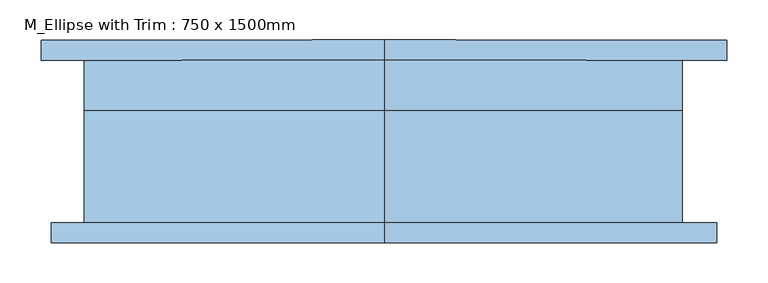
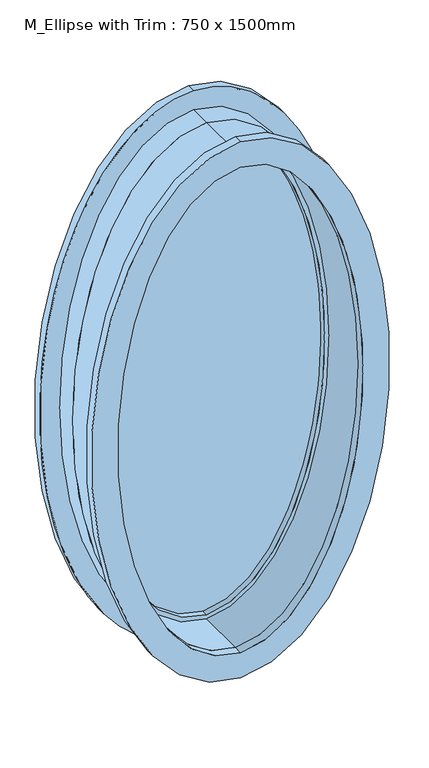
"""IFC4 building model written with IfcOpenShell, lengths in millimetres: window geometry, M_Ellipse with Trim : 750 x 1500mm."""

import ifcopenshell
import ifcopenshell.guid

model = None  # the IFC model being written
_history = None  # IfcOwnerHistory: only IFC2X3 demands one
_inside = {}  # id of a spatial element -> (the spatial element, [elements in it])
_under = {}  # id of a project, library or spatial element -> (it, [spatial elements below it])
_declared = {}  # id of a project -> (the project, [libraries it declares])
_typed = {}  # id of a type object -> (the type object, [elements of that type])
_made_of = {}  # id of a material, layer set ... -> (it, [elements and type objects made of it])


def new_model(schema):
    """Start an empty IFC model of exactly this schema.

    Asked for "IFC4X3", IfcOpenShell would pick the latest addendum, in which some entities
    have other attributes; the version numbers below select the first issue.
    IFC2X3 requires an IfcOwnerHistory on every rooted entity: one is made here for all.
    """
    global model, _history
    if schema == "IFC4X3":
        model = ifcopenshell.file(schema_version=(4, 3, 0, 0))
    else:
        model = ifcopenshell.file(schema=schema)
    _inside.clear()
    _under.clear()
    _declared.clear()
    _typed.clear()
    _made_of.clear()
    _history = None
    if model.schema == "IFC2X3":
        org = make("IfcOrganization", Name="unknown")
        user = make(
            "IfcPersonAndOrganization",
            ThePerson=make("IfcPerson", FamilyName="unknown"),
            TheOrganization=org,
        )
        app = make(
            "IfcApplication",
            ApplicationDeveloper=org,
            Version="unknown",
            ApplicationFullName="unknown",
            ApplicationIdentifier="unknown",
        )
        _history = make(
            "IfcOwnerHistory",
            OwningUser=user,
            OwningApplication=app,
            ChangeAction="ADDED",
            CreationDate=0,
        )
    return model


def make(cls, **values):
    """One entity of the class cls with the attributes given. An attribute that is None is left unset."""
    return model.create_entity(
        cls, **{name: value for name, value in values.items() if value is not None}
    )


def rooted(cls, **values):
    """An entity with a GlobalId (a new one), such as an element, a storey or a relation."""
    return make(cls, GlobalId=ifcopenshell.guid.new(), OwnerHistory=_history, **values)


def si_unit(unit_type, name, prefix=None):
    """IfcSIUnit, for example si_unit("LENGTHUNIT", "METRE", prefix="MILLI")."""
    return make("IfcSIUnit", UnitType=unit_type, Prefix=prefix, Name=name)


def assignment(units):
    """IfcUnitAssignment: the units of a project."""
    return None if units is None else make("IfcUnitAssignment", Units=units)


def point(xyz):
    """IfcCartesianPoint."""
    return None if xyz is None else make("IfcCartesianPoint", Coordinates=xyz)


def direction(xyz):
    """IfcDirection."""
    return None if xyz is None else make("IfcDirection", DirectionRatios=xyz)


def frame(location, z_axis=None, x_axis=None):
    """IfcAxis2Placement3D, a coordinate frame: its origin and axes. An axis left out is left unset."""
    return make(
        "IfcAxis2Placement3D",
        Location=point(location),
        Axis=direction(z_axis),
        RefDirection=direction(x_axis),
    )


def origin():
    """The frame at (0, 0, 0) with its axes left unset."""
    return frame((0.0, 0.0, 0.0))


def place(relative_to, where):
    """IfcLocalPlacement: puts the frame where relative to a parent placement (None: the world)."""
    return make(
        "IfcLocalPlacement", PlacementRelTo=relative_to, RelativePlacement=where
    )


def context(
    kind, dimensions, precision=None, world=None, true_north=None, identifier=None
):
    """IfcGeometricRepresentationContext, for example the 3D "Model" context."""
    return make(
        "IfcGeometricRepresentationContext",
        ContextIdentifier=identifier,
        ContextType=kind,
        CoordinateSpaceDimension=dimensions,
        Precision=precision,
        WorldCoordinateSystem=world,
        TrueNorth=true_north,
    )


def project(units=None, contexts=None):
    """IfcProject with its units and contexts."""
    return rooted(
        "IfcProject",
        Name="project",
        RepresentationContexts=contexts,
        UnitsInContext=assignment(units),
    )


def spatial(cls, under=None, at=None, **own):
    """A site, building, storey or space (cls), placed at a placement, below another one or the project."""
    s = rooted(cls, ObjectPlacement=at, **own)
    if under is not None:
        _under.setdefault(under.id(), (under, []))[1].append(s)
    return s


def ellipse_curve(where, semi_axis1, semi_axis2):
    """IfcEllipse in the frame where."""
    return make(
        "IfcEllipse", Position=where, SemiAxis1=semi_axis1, SemiAxis2=semi_axis2
    )


def trimmed(basis, trim1, trim2, sense, master):
    """IfcTrimmedCurve: the piece of a basis curve between two trims."""
    return make(
        "IfcTrimmedCurve",
        BasisCurve=basis,
        Trim1=trim1,
        Trim2=trim2,
        SenseAgreement=sense,
        MasterRepresentation=master,
    )


def shape(context_of_items, identifier, shape_type, items):
    """IfcShapeRepresentation: the items that make up one representation, for example the "Body"."""
    return make(
        "IfcShapeRepresentation",
        ContextOfItems=context_of_items,
        RepresentationIdentifier=identifier,
        RepresentationType=shape_type,
        Items=items,
    )


def source(mapping_origin, context_of_items, identifier, shape_type, items):
    """IfcRepresentationMap: a shape defined once, which mapped items show again and again."""
    return make(
        "IfcRepresentationMap",
        MappingOrigin=mapping_origin,
        MappedRepresentation=shape(context_of_items, identifier, shape_type, items),
    )


def transform(
    local_origin,
    x_axis=None,
    y_axis=None,
    z_axis=None,
    scale=None,
    scale2=None,
    scale3=None,
    uniform=True,
):
    """IfcCartesianTransformationOperator3D, or its non-uniform kind. x_axis, y_axis, z_axis: its Axis1, 2, 3."""
    if uniform:
        return make(
            "IfcCartesianTransformationOperator3D",
            Axis1=direction(x_axis),
            Axis2=direction(y_axis),
            LocalOrigin=point(local_origin),
            Scale=scale,
            Axis3=direction(z_axis),
        )
    return make(
        "IfcCartesianTransformationOperator3DnonUniform",
        Axis1=direction(x_axis),
        Axis2=direction(y_axis),
        LocalOrigin=point(local_origin),
        Scale=scale,
        Axis3=direction(z_axis),
        Scale2=scale2,
        Scale3=scale3,
    )


def mapped(mapping_source, mapping_target):
    """IfcMappedItem: shows the shape of a source again, moved by a transform."""
    return make(
        "IfcMappedItem", MappingSource=mapping_source, MappingTarget=mapping_target
    )


def made_of(thing, what):
    """Note that an element or type object is made of a material, layer set ...; save() writes the relation."""
    if what is not None:
        _made_of.setdefault(what.id(), (what, []))[1].append(thing)
    return thing


def element(
    cls,
    number,
    at=None,
    inside=None,
    cuts=None,
    type_object=None,
    material=None,
    context=None,
    identifier="Body",
    shape_type=None,
    held_by="IfcProductDefinitionShape",
    body=None,
    shapes=None,
    **own,
):
    """One element of the class cls, such as IfcWall. Its Tag is "e" and its number.

    at: its placement. inside: the storey or other place that contains it. cuts: it is an
    opening in that element (IfcRelVoidsElement). A single representation is given by context,
    identifier, shape_type and body (its items); several are given by shapes. held_by: the class
    of the entity that holds the representations. save() writes the other relations.
    """
    e = rooted(cls, Tag="e%d" % number, ObjectPlacement=at, **own)
    if body is not None:
        shapes = [shape(context, identifier, shape_type, body)]
    if shapes is not None:
        e.Representation = make(held_by, Representations=shapes)
    if inside is not None:
        _inside.setdefault(inside.id(), (inside, []))[1].append(e)
    if cuts is not None:
        rooted(
            "IfcRelVoidsElement", RelatingBuildingElement=cuts, RelatedOpeningElement=e
        )
    if type_object is not None:
        _typed.setdefault(type_object.id(), (type_object, []))[1].append(e)
    return made_of(e, material)


def aggregate(whole, parts):
    """IfcRelAggregates: a whole, such as a stair, and the parts it consists of."""
    return rooted("IfcRelAggregates", RelatingObject=whole, RelatedObjects=parts)


def save(model, path):
    """Write the relations noted so far, then the file.

    IfcRelAggregates (storeys below a building ...), IfcRelContainedInSpatialStructure (elements
    in a storey), IfcRelDefinesByType, IfcRelAssociatesMaterial and IfcRelDeclares: one each for
    every whole, place, type object, material and project.
    """
    for whole, parts in _under.values():
        aggregate(whole, parts)
    for where, things in _inside.values():
        rooted(
            "IfcRelContainedInSpatialStructure",
            RelatedElements=things,
            RelatingStructure=where,
        )
    for kind, things in _typed.values():
        rooted("IfcRelDefinesByType", RelatedObjects=things, RelatingType=kind)
    for what, things in _made_of.values():
        rooted("IfcRelAssociatesMaterial", RelatedObjects=things, RelatingMaterial=what)
    for by, libraries in _declared.values():
        rooted("IfcRelDeclares", RelatingContext=by, RelatedDefinitions=libraries)
    model.write(path)


def plane_surface(at):
    """IfcPlane: the flat surface through the origin of the frame at, square to its z axis."""
    return make("IfcPlane", Position=at)


def extruded_surface(curve, direction_of_extrusion, depth):
    """IfcSurfaceOfLinearExtrusion: the curve pushed along a direction by depth."""
    return make(
        "IfcSurfaceOfLinearExtrusion",
        SweptCurve=make("IfcArbitraryOpenProfileDef", ProfileType="CURVE", Curve=curve),
        ExtrudedDirection=direction(direction_of_extrusion),
        Depth=depth,
    )


def advanced_brep(points, edges, surfaces, faces):
    """IfcAdvancedBrep: a solid bounded by faces that lie on surfaces and meet in shared edges.

    An edge is (start, end): straight between two places in points (the first is 0);
    or (start, end, curve); or (start, end, curve, False) where it runs against its curve.
    A face is (place in surfaces, loops), or (place, loops, False) where it looks against
    its surface's normal. A loop lists edges by number (the first is 1), with a minus sign
    where the edge is run from its end to its start. The first loop is the outer one.
    """
    corners = [point(p) for p in points]
    vertices = [make("IfcVertexPoint", VertexGeometry=c) for c in corners]
    made = []
    for start, end, *more in edges:
        made.append(
            make(
                "IfcEdgeCurve",
                EdgeStart=vertices[start],
                EdgeEnd=vertices[end],
                EdgeGeometry=more[0] if more else make("IfcPolyline", Points=[corners[start], corners[end]]),
                SameSense=more[1] if len(more) > 1 else True,
            )
        )
    hull = []
    for where, loops, *sense in faces:
        bounds = []
        for j, loop in enumerate(loops):
            ring = [make("IfcOrientedEdge", EdgeElement=made[abs(k) - 1], Orientation=k > 0) for k in loop]
            bounds.append(
                make(
                    "IfcFaceOuterBound" if j == 0 else "IfcFaceBound",
                    Bound=make("IfcEdgeLoop", EdgeList=ring),
                    Orientation=True,
                )
            )
        hull.append(make("IfcAdvancedFace", Bounds=bounds, FaceSurface=surfaces[where], SameSense=sense[0] if sense else True))
    return make("IfcAdvancedBrep", Outer=make("IfcClosedShell", CfsFaces=hull))


def m_ellipse_with_trim_750_x_1500mm_90dfdbfc(model_context):
    return source(origin(), model_context, "Body", "AdvancedBrep", [
        advanced_brep(
        [(0.0, -101.6, 2415.0), (0.0, -101.6, 915.0), (0.0, -101.6, 2383.25), (0.0, -101.6, 946.75), (0.0, 38.1, 2415.0), (0.0, 38.1, 915.0), (0.0, 38.1, 2383.25), (0.0, 38.1, 946.75)],
        [
            (0, 1, ellipse_curve(frame((0.0, -101.6, 1665.0), z_axis=(0.0, -1.0, 0.0), x_axis=(0.0, 0.0, -1.0)), 750.0, 375.0)),
            (1, 0, ellipse_curve(frame((0.0, -101.6, 1665.0), z_axis=(0.0, -1.0, 0.0), x_axis=(0.0, 0.0, -1.0)), 750.0, 375.0)),
            (2, 3, ellipse_curve(frame((0.0, -101.6, 1665.0), z_axis=(0.0, 1.0, 0.0), x_axis=(0.0, 0.0, -1.0)), 718.25, 343.25)),
            (3, 2, ellipse_curve(frame((0.0, -101.6, 1665.0), z_axis=(0.0, 1.0, 0.0), x_axis=(0.0, 0.0, -1.0)), 718.25, 343.25)),
            (0, 4),
            (4, 5, ellipse_curve(frame((0.0, 38.1, 1665.0), z_axis=(0.0, -1.0, 0.0), x_axis=(0.0, 0.0, -1.0)), 750.0, 375.0)),
            (5, 1),
            (5, 4, ellipse_curve(frame((0.0, 38.1, 1665.0), z_axis=(0.0, -1.0, 0.0), x_axis=(0.0, 0.0, -1.0)), 750.0, 375.0)),
            (2, 6),
            (6, 7, ellipse_curve(frame((0.0, 38.1, 1665.0), z_axis=(0.0, 1.0, 0.0), x_axis=(0.0, 0.0, -1.0)), 718.25, 343.25)),
            (7, 3),
            (7, 6, ellipse_curve(frame((0.0, 38.1, 1665.0), z_axis=(0.0, 1.0, 0.0), x_axis=(0.0, 0.0, -1.0)), 718.25, 343.25)),
        ],
        [
            plane_surface(frame((0.0, -101.6, 915.0), z_axis=(0.0, -1.0, 0.0), x_axis=(1.0, 0.0, 0.0))),
            extruded_surface(trimmed(ellipse_curve(frame((0.0, 177.8, 1665.0), z_axis=(0.0, -1.0, 0.0), x_axis=(0.0, 0.0, -1.0)), 750.0, 375.0), [point((0.0, 177.8, 2415.0))], [point((0.0, 177.8, 915.0))], True, "CARTESIAN"), (0.0, -139.70000000000002, 0.0), 139.70000000000002),
            extruded_surface(trimmed(ellipse_curve(frame((0.0, 177.8, 1665.0), z_axis=(0.0, -1.0, 0.0), x_axis=(0.0, 0.0, -1.0)), 750.0, 375.0), [point((0.0, 177.8, 915.0))], [point((0.0, 177.8, 2415.0))], True, "CARTESIAN"), (0.0, -139.70000000000002, 0.0), 139.70000000000002),
            extruded_surface(trimmed(ellipse_curve(frame((0.0, 38.1, 1665.0), z_axis=(0.0, 1.0, 0.0), x_axis=(0.0, 0.0, -1.0)), 718.25, 343.25), [point((0.0, 38.1, 2383.25))], [point((0.0, 38.1, 946.75))], True, "CARTESIAN"), (0.0, -139.7, 0.0), 139.7),
            extruded_surface(trimmed(ellipse_curve(frame((0.0, 38.1, 1665.0), z_axis=(0.0, 1.0, 0.0), x_axis=(0.0, 0.0, -1.0)), 718.25, 343.25), [point((0.0, 38.1, 946.75))], [point((0.0, 38.1, 2383.25))], True, "CARTESIAN"), (0.0, -139.7, 0.0), 139.7),
            plane_surface(frame((0.0, 38.1, 915.0), z_axis=(0.0, 1.0, 0.0), x_axis=(-1.0, 0.0, 0.0))),
        ],
        [
            (0, [[1, 2], [3, 4]]),
            (1, [[-1, 5, 6, 7]]),
            (2, [[-2, -7, 8, -5]]),
            (3, [[-3, 9, 10, 11]]),
            (4, [[-4, -11, 12, -9]]),
            (5, [[-8, -6], [-12, -10]]),
        ],
    ),
        advanced_brep(
        [(0.0, 55.3459129, 2370.55), (0.0, 55.3459129, 959.45), (0.0, 64.8706843, 2370.55), (0.0, 64.8706843, 959.45)],
        [
            (0, 1, ellipse_curve(frame((0.0, 55.3459129, 1665.0), z_axis=(0.0, -1.0, 0.0), x_axis=(0.0, 0.0, -1.0)), 705.55, 330.55)),
            (1, 0, ellipse_curve(frame((0.0, 55.3459129, 1665.0), z_axis=(0.0, -1.0, 0.0), x_axis=(0.0, 0.0, -1.0)), 705.55, 330.55)),
            (0, 2),
            (2, 3, ellipse_curve(frame((0.0, 64.8706843, 1665.0), z_axis=(0.0, -1.0, 0.0), x_axis=(0.0, 0.0, -1.0)), 705.55, 330.55)),
            (3, 1),
            (3, 2, ellipse_curve(frame((0.0, 64.8706843, 1665.0), z_axis=(0.0, -1.0, 0.0), x_axis=(0.0, 0.0, -1.0)), 705.55, 330.55)),
        ],
        [
            plane_surface(frame((0.0, 55.3459129, 959.45), z_axis=(0.0, -1.0, 0.0), x_axis=(1.0, 0.0, 0.0))),
            extruded_surface(trimmed(ellipse_curve(frame((0.0, 74.3954558, 1665.0), z_axis=(0.0, -1.0, 0.0), x_axis=(0.0, 0.0, -1.0)), 705.55, 330.55), [point((0.0, 74.3954558, 2370.55))], [point((0.0, 74.3954558, 959.45))], True, "CARTESIAN"), (0.0, -9.5247715, 0.0), 9.5247715),
            extruded_surface(trimmed(ellipse_curve(frame((0.0, 74.3954558, 1665.0), z_axis=(0.0, -1.0, 0.0), x_axis=(0.0, 0.0, -1.0)), 705.55, 330.55), [point((0.0, 74.3954558, 959.45))], [point((0.0, 74.3954558, 2370.55))], True, "CARTESIAN"), (0.0, -9.5247715, 0.0), 9.5247715),
            plane_surface(frame((0.0, 64.8706843, 959.45), z_axis=(0.0, 1.0, 0.0), x_axis=(-1.0, 0.0, 0.0))),
        ],
        [
            (0, [[1, 2]]),
            (1, [[-1, 3, 4, 5]]),
            (2, [[-2, -5, 6, -3]]),
            (3, [[-6, -4]]),
        ],
    ),
        advanced_brep(
        [(0.0, 38.1, 2395.95), (0.0, 38.1, 934.05), (0.0, 38.1, 2370.55), (0.0, 38.1, 959.45), (0.0, 82.55, 2395.95), (0.0, 82.55, 934.05), (0.0, 82.55, 2370.55), (0.0, 82.55, 959.45)],
        [
            (0, 1, ellipse_curve(frame((0.0, 38.1, 1665.0), z_axis=(0.0, -1.0, 0.0), x_axis=(0.0, 0.0, -1.0)), 730.95, 355.95)),
            (1, 0, ellipse_curve(frame((0.0, 38.1, 1665.0), z_axis=(0.0, -1.0, 0.0), x_axis=(0.0, 0.0, -1.0)), 730.95, 355.95)),
            (2, 3, ellipse_curve(frame((0.0, 38.1, 1665.0), z_axis=(0.0, 1.0, 0.0), x_axis=(0.0, 0.0, -1.0)), 705.55, 330.55)),
            (3, 2, ellipse_curve(frame((0.0, 38.1, 1665.0), z_axis=(0.0, 1.0, 0.0), x_axis=(0.0, 0.0, -1.0)), 705.55, 330.55)),
            (0, 4),
            (4, 5, ellipse_curve(frame((0.0, 82.55, 1665.0), z_axis=(0.0, -1.0, 0.0), x_axis=(0.0, 0.0, -1.0)), 730.95, 355.95)),
            (5, 1),
            (5, 4, ellipse_curve(frame((0.0, 82.55, 1665.0), z_axis=(0.0, -1.0, 0.0), x_axis=(0.0, 0.0, -1.0)), 730.95, 355.95)),
            (2, 6),
            (6, 7, ellipse_curve(frame((0.0, 82.55, 1665.0), z_axis=(0.0, 1.0, 0.0), x_axis=(0.0, 0.0, -1.0)), 705.55, 330.55)),
            (7, 3),
            (7, 6, ellipse_curve(frame((0.0, 82.55, 1665.0), z_axis=(0.0, 1.0, 0.0), x_axis=(0.0, 0.0, -1.0)), 705.55, 330.55)),
        ],
        [
            plane_surface(frame((0.0, 38.1, 934.05), z_axis=(0.0, -1.0, 0.0), x_axis=(1.0, 0.0, 0.0))),
            extruded_surface(trimmed(ellipse_curve(frame((0.0, 127.0, 1665.0), z_axis=(0.0, -1.0, 0.0), x_axis=(0.0, 0.0, -1.0)), 730.95, 355.95), [point((0.0, 127.0, 2395.95))], [point((0.0, 127.0, 934.05))], True, "CARTESIAN"), (0.0, -44.45, 0.0), 44.45),
            extruded_surface(trimmed(ellipse_curve(frame((0.0, 127.0, 1665.0), z_axis=(0.0, -1.0, 0.0), x_axis=(0.0, 0.0, -1.0)), 730.95, 355.95), [point((0.0, 127.0, 934.05))], [point((0.0, 127.0, 2395.95))], True, "CARTESIAN"), (0.0, -44.45, 0.0), 44.45),
            extruded_surface(trimmed(ellipse_curve(frame((0.0, 146.05, 1665.0), z_axis=(0.0, 1.0, 0.0), x_axis=(0.0, 0.0, -1.0)), 705.55, 330.55), [point((0.0, 146.05, 2370.55))], [point((0.0, 146.05, 959.45))], True, "CARTESIAN"), (0.0, -44.45000000000002, 0.0), 44.45000000000002),
            extruded_surface(trimmed(ellipse_curve(frame((0.0, 146.05, 1665.0), z_axis=(0.0, 1.0, 0.0), x_axis=(0.0, 0.0, -1.0)), 705.55, 330.55), [point((0.0, 146.05, 959.45))], [point((0.0, 146.05, 2370.55))], True, "CARTESIAN"), (0.0, -44.45000000000002, 0.0), 44.45000000000002),
            plane_surface(frame((0.0, 82.55, 934.05), z_axis=(0.0, 1.0, 0.0), x_axis=(-1.0, 0.0, 0.0))),
        ],
        [
            (0, [[1, 2], [3, 4]]),
            (1, [[-1, 5, 6, 7]]),
            (2, [[-2, -7, 8, -5]]),
            (3, [[-3, 9, 10, 11]]),
            (4, [[-4, -11, 12, -9]]),
            (5, [[-8, -6], [-12, -10]]),
        ],
    ),
        advanced_brep(
        [(0.0, 38.1, 2415.0), (0.0, 38.1, 915.0), (0.0, 38.1, 2395.95), (0.0, 38.1, 934.05), (0.0, 101.6, 2415.0), (0.0, 101.6, 915.0), (0.0, 101.6, 2395.95), (0.0, 101.6, 934.05)],
        [
            (0, 1, ellipse_curve(frame((0.0, 38.1, 1665.0), z_axis=(0.0, -1.0, 0.0), x_axis=(0.0, 0.0, -1.0)), 750.0, 375.0)),
            (1, 0, ellipse_curve(frame((0.0, 38.1, 1665.0), z_axis=(0.0, -1.0, 0.0), x_axis=(0.0, 0.0, -1.0)), 750.0, 375.0)),
            (2, 3, ellipse_curve(frame((0.0, 38.1, 1665.0), z_axis=(0.0, 1.0, 0.0), x_axis=(0.0, 0.0, -1.0)), 730.95, 355.95)),
            (3, 2, ellipse_curve(frame((0.0, 38.1, 1665.0), z_axis=(0.0, 1.0, 0.0), x_axis=(0.0, 0.0, -1.0)), 730.95, 355.95)),
            (0, 4),
            (4, 5, ellipse_curve(frame((0.0, 101.6, 1665.0), z_axis=(0.0, -1.0, 0.0), x_axis=(0.0, 0.0, -1.0)), 750.0, 375.0)),
            (5, 1),
            (5, 4, ellipse_curve(frame((0.0, 101.6, 1665.0), z_axis=(0.0, -1.0, 0.0), x_axis=(0.0, 0.0, -1.0)), 750.0, 375.0)),
            (2, 6),
            (6, 7, ellipse_curve(frame((0.0, 101.6, 1665.0), z_axis=(0.0, 1.0, 0.0), x_axis=(0.0, 0.0, -1.0)), 730.95, 355.95)),
            (7, 3),
            (7, 6, ellipse_curve(frame((0.0, 101.6, 1665.0), z_axis=(0.0, 1.0, 0.0), x_axis=(0.0, 0.0, -1.0)), 730.95, 355.95)),
        ],
        [
            plane_surface(frame((0.0, 38.1, 915.0), z_axis=(0.0, -1.0, 0.0), x_axis=(1.0, 0.0, 0.0))),
            extruded_surface(trimmed(ellipse_curve(frame((0.0, 165.1, 1665.0), z_axis=(0.0, -1.0, 0.0), x_axis=(0.0, 0.0, -1.0)), 750.0, 375.0), [point((0.0, 165.1, 2415.0))], [point((0.0, 165.1, 915.0))], True, "CARTESIAN"), (0.0, -63.5, 0.0), 63.5),
            extruded_surface(trimmed(ellipse_curve(frame((0.0, 165.1, 1665.0), z_axis=(0.0, -1.0, 0.0), x_axis=(0.0, 0.0, -1.0)), 750.0, 375.0), [point((0.0, 165.1, 915.0))], [point((0.0, 165.1, 2415.0))], True, "CARTESIAN"), (0.0, -63.5, 0.0), 63.5),
            extruded_surface(trimmed(ellipse_curve(frame((0.0, 165.1, 1665.0), z_axis=(0.0, 1.0, 0.0), x_axis=(0.0, 0.0, -1.0)), 730.95, 355.95), [point((0.0, 165.1, 2395.95))], [point((0.0, 165.1, 934.05))], True, "CARTESIAN"), (0.0, -63.5, 0.0), 63.5),
            extruded_surface(trimmed(ellipse_curve(frame((0.0, 165.1, 1665.0), z_axis=(0.0, 1.0, 0.0), x_axis=(0.0, 0.0, -1.0)), 730.95, 355.95), [point((0.0, 165.1, 934.05))], [point((0.0, 165.1, 2395.95))], True, "CARTESIAN"), (0.0, -63.5, 0.0), 63.5),
            plane_surface(frame((0.0, 101.6, 915.0), z_axis=(0.0, 1.0, 0.0), x_axis=(-1.0, 0.0, 0.0))),
        ],
        [
            (0, [[1, 2], [3, 4]]),
            (1, [[-1, 5, 6, 7]]),
            (2, [[-2, -7, 8, -5]]),
            (3, [[-3, 9, 10, 11]]),
            (4, [[-4, -11, 12, -9]]),
            (5, [[-8, -6], [-12, -10]]),
        ],
    ),
        advanced_brep(
        [(0.0, -126.6, 2458.25), (0.0, -126.6, 871.75), (0.0, -126.6, 2383.25), (0.0, -126.6, 946.75), (0.0, -101.6, 2458.25), (0.0, -101.6, 871.75), (0.0, -101.6, 2383.25), (0.0, -101.6, 946.75)],
        [
            (0, 1, ellipse_curve(frame((0.0, -126.6, 1665.0), z_axis=(0.0, -1.0, 0.0), x_axis=(0.0, 0.0, -1.0)), 793.25, 418.25)),
            (1, 0, ellipse_curve(frame((0.0, -126.6, 1665.0), z_axis=(0.0, -1.0, 0.0), x_axis=(0.0, 0.0, -1.0)), 793.25, 418.25)),
            (2, 3, ellipse_curve(frame((0.0, -126.6, 1665.0), z_axis=(0.0, 1.0, 0.0), x_axis=(0.0, 0.0, -1.0)), 718.25, 343.25)),
            (3, 2, ellipse_curve(frame((0.0, -126.6, 1665.0), z_axis=(0.0, 1.0, 0.0), x_axis=(0.0, 0.0, -1.0)), 718.25, 343.25)),
            (4, 5, ellipse_curve(frame((0.0, -101.6, 1665.0), z_axis=(0.0, 1.0, 0.0), x_axis=(0.0, 0.0, -1.0)), 793.25, 418.25)),
            (5, 4, ellipse_curve(frame((0.0, -101.6, 1665.0), z_axis=(0.0, 1.0, 0.0), x_axis=(0.0, 0.0, -1.0)), 793.25, 418.25)),
            (6, 7, ellipse_curve(frame((0.0, -101.6, 1665.0), z_axis=(0.0, -1.0, 0.0), x_axis=(0.0, 0.0, -1.0)), 718.25, 343.25)),
            (7, 6, ellipse_curve(frame((0.0, -101.6, 1665.0), z_axis=(0.0, -1.0, 0.0), x_axis=(0.0, 0.0, -1.0)), 718.25, 343.25)),
            (2, 6),
            (7, 3),
            (0, 4),
            (5, 1),
        ],
        [
            plane_surface(frame((0.0, -126.6, 946.75), z_axis=(0.0, -1.0, 0.0), x_axis=(-1.0, 0.0, 0.0))),
            plane_surface(frame((0.0, -101.6, 946.75), z_axis=(0.0, 1.0, 0.0), x_axis=(1.0, 0.0, 0.0))),
            extruded_surface(trimmed(ellipse_curve(frame((0.0, -76.6, 1665.0), z_axis=(0.0, 1.0, 0.0), x_axis=(0.0, 0.0, -1.0)), 718.25, 343.25), [point((0.0, -76.6, 2383.25))], [point((0.0, -76.6, 946.75))], True, "CARTESIAN"), (0.0, -25.0, 0.0), 25.0),
            extruded_surface(trimmed(ellipse_curve(frame((0.0, -76.6, 1665.0), z_axis=(0.0, 1.0, 0.0), x_axis=(0.0, 0.0, -1.0)), 718.25, 343.25), [point((0.0, -76.6, 946.75))], [point((0.0, -76.6, 2383.25))], True, "CARTESIAN"), (0.0, -25.0, 0.0), 25.0),
            extruded_surface(trimmed(ellipse_curve(frame((0.0, -76.6, 1665.0), z_axis=(0.0, -1.0, 0.0), x_axis=(0.0, 0.0, -1.0)), 793.25, 418.25), [point((0.0, -76.6, 2458.25))], [point((0.0, -76.6, 871.75))], True, "CARTESIAN"), (0.0, -25.0, 0.0), 25.0),
            extruded_surface(trimmed(ellipse_curve(frame((0.0, -76.6, 1665.0), z_axis=(0.0, -1.0, 0.0), x_axis=(0.0, 0.0, -1.0)), 793.25, 418.25), [point((0.0, -76.6, 871.75))], [point((0.0, -76.6, 2458.25))], True, "CARTESIAN"), (0.0, -25.0, 0.0), 25.0),
        ],
        [
            (0, [[1, 2], [3, 4]]),
            (1, [[5, 6], [7, 8]]),
            (2, [[-3, 9, -8, 10]]),
            (3, [[-4, -10, -7, -9]]),
            (4, [[-1, 11, -6, 12]]),
            (5, [[-2, -12, -5, -11]]),
        ],
    ),
        advanced_brep(
        [(0.0, 101.6, 2470.95), (0.0, 101.6, 859.05), (0.0, 101.6, 2395.95), (0.0, 101.6, 934.05), (0.0, 126.6, 2470.95), (0.0, 126.6, 859.05), (0.0, 126.6, 2395.95), (0.0, 126.6, 934.05)],
        [
            (0, 1, ellipse_curve(frame((0.0, 101.6, 1665.0), z_axis=(0.0, -1.0, 0.0), x_axis=(0.0, 0.0, -1.0)), 805.95, 430.95)),
            (1, 0, ellipse_curve(frame((0.0, 101.6, 1665.0), z_axis=(0.0, -1.0, 0.0), x_axis=(0.0, 0.0, -1.0)), 805.95, 430.95)),
            (2, 3, ellipse_curve(frame((0.0, 101.6, 1665.0), z_axis=(0.0, 1.0, 0.0), x_axis=(0.0, 0.0, -1.0)), 730.95, 355.95)),
            (3, 2, ellipse_curve(frame((0.0, 101.6, 1665.0), z_axis=(0.0, 1.0, 0.0), x_axis=(0.0, 0.0, -1.0)), 730.95, 355.95)),
            (4, 5, ellipse_curve(frame((0.0, 126.6, 1665.0), z_axis=(0.0, 1.0, 0.0), x_axis=(0.0, 0.0, -1.0)), 805.95, 430.95)),
            (5, 4, ellipse_curve(frame((0.0, 126.6, 1665.0), z_axis=(0.0, 1.0, 0.0), x_axis=(0.0, 0.0, -1.0)), 805.95, 430.95)),
            (6, 7, ellipse_curve(frame((0.0, 126.6, 1665.0), z_axis=(0.0, -1.0, 0.0), x_axis=(0.0, 0.0, -1.0)), 730.95, 355.95)),
            (7, 6, ellipse_curve(frame((0.0, 126.6, 1665.0), z_axis=(0.0, -1.0, 0.0), x_axis=(0.0, 0.0, -1.0)), 730.95, 355.95)),
            (2, 6),
            (7, 3),
            (0, 4),
            (5, 1),
        ],
        [
            plane_surface(frame((0.0, 101.6, 934.05), z_axis=(0.0, -1.0, 0.0), x_axis=(-1.0, 0.0, 0.0))),
            plane_surface(frame((0.0, 126.6, 934.05), z_axis=(0.0, 1.0, 0.0), x_axis=(1.0, 0.0, 0.0))),
            extruded_surface(trimmed(ellipse_curve(frame((0.0, 151.6, 1665.0), z_axis=(0.0, 1.0, 0.0), x_axis=(0.0, 0.0, -1.0)), 730.95, 355.95), [point((0.0, 151.6, 2395.95))], [point((0.0, 151.6, 934.05))], True, "CARTESIAN"), (0.0, -25.0, 0.0), 25.0),
            extruded_surface(trimmed(ellipse_curve(frame((0.0, 151.6, 1665.0), z_axis=(0.0, 1.0, 0.0), x_axis=(0.0, 0.0, -1.0)), 730.95, 355.95), [point((0.0, 151.6, 934.05))], [point((0.0, 151.6, 2395.95))], True, "CARTESIAN"), (0.0, -25.0, 0.0), 25.0),
            extruded_surface(trimmed(ellipse_curve(frame((0.0, 126.6, 1665.0), z_axis=(0.0, -1.0, 0.0), x_axis=(0.0, 0.0, -1.0)), 805.95, 430.95), [point((0.0, 126.6, 2470.95))], [point((0.0, 126.6, 859.05))], True, "CARTESIAN"), (0.0, -25.0, 0.0), 25.0),
            extruded_surface(trimmed(ellipse_curve(frame((0.0, 126.6, 1665.0), z_axis=(0.0, -1.0, 0.0), x_axis=(0.0, 0.0, -1.0)), 805.95, 430.95), [point((0.0, 126.6, 859.05))], [point((0.0, 126.6, 2470.95))], True, "CARTESIAN"), (0.0, -25.0, 0.0), 25.0),
        ],
        [
            (0, [[1, 2], [3, 4]]),
            (1, [[5, 6], [7, 8]]),
            (2, [[-3, 9, -8, 10]]),
            (3, [[-4, -10, -7, -9]]),
            (4, [[-1, 11, -6, 12]]),
            (5, [[-2, -12, -5, -11]]),
        ],
    ),
    ])


if __name__ == "__main__":
    model = new_model("IFC4")
    model_context = context("Model", 3, world=origin())
    ifc_project = project(units=[si_unit("LENGTHUNIT", "METRE", prefix="MILLI")], contexts=[model_context])
    site = spatial("IfcSite", under=ifc_project)
    building = spatial("IfcBuilding", under=site)
    placement = place(None, origin())
    m_ellipse_with_trim_750_x_1500mm_shape = m_ellipse_with_trim_750_x_1500mm_90dfdbfc(model_context)
    element("IfcWindow", 1, ObjectType="M_Ellipse with Trim : 750 x 1500mm", at=placement, inside=building, context=model_context, shape_type="MappedRepresentation", body=[
        mapped(m_ellipse_with_trim_750_x_1500mm_shape, transform((0.0, 0.0, 0.0), x_axis=(1.0, 0.0, 0.0), y_axis=(0.0, 1.0, 0.0), z_axis=(0.0, 0.0, 1.0))),
    ])
    save(model, "model.ifc")

# Revit data of these elements
# Type "M_Ellipse with Trim : 750 x 1500mm"
#   Type Mark = "20"
#   Construction Type Id = "GSP4R"
#   Analytic Construction = "1/8 in Pilkington single glazing"
#   Visual Light Transmittance = 0.9
#   Thermal Resistance (R) = 0.1491 (m²·K)/W
#   Solar Heat Gain Coefficient = 0.86
#   Height = 4' - 11.05512"
#   Heat Transfer Coefficient (U) = 6.7069 W/(m²·K)
#   Half Width = 1' - 2.76378"
#   Half Height = 2' - 5.52756"
#   Default Sill Height = 3' - 0.02362"
#   Trim Projection = 0' - 0.98425"
#   Trim Width = 0' - 2.95276"
#   Width = 2' - 5.52756"
#   Trim Material = none
#   Sash Material = none
#   Wall Closure = (empty or 0)
# Element 1 (IfcWindow, "M_Ellipse with Trim : 750 x 1500mm")
#   Materials on its faces: "Glass"
# Materials
#   "Glass": class "Glass", colour RGB 0 128 192, transparency 0.75, Description = "Soda Lime Glass", Cost = 0
